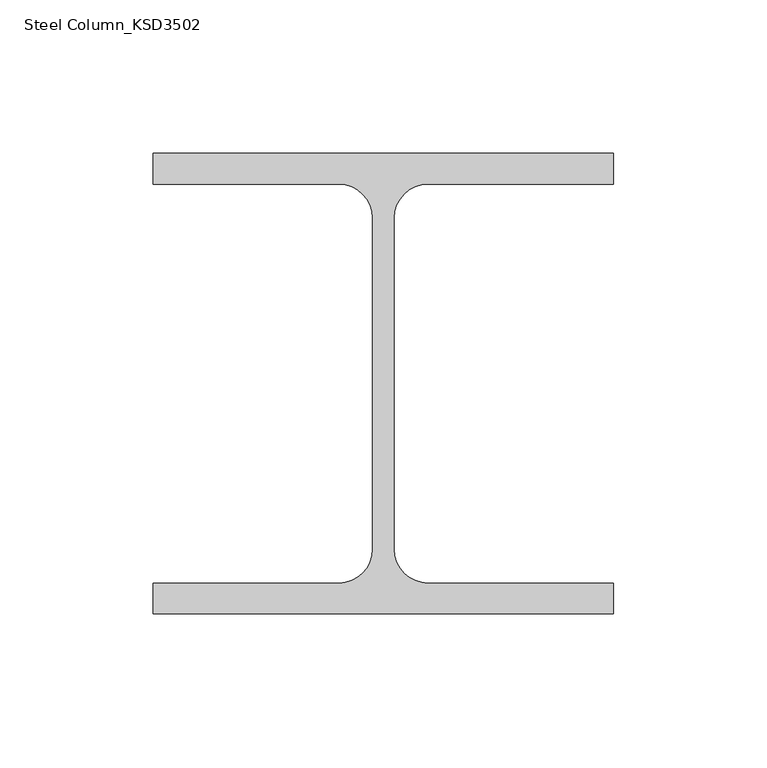
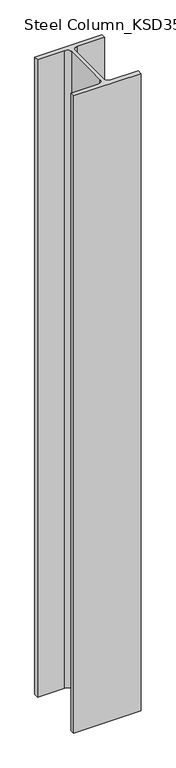
"""IFC4 building model written with IfcOpenShell, lengths in millimetres: column geometry, Steel Column_KSD3502 : H_SC_ASC_H-150×150x7x10."""

from ifc_helpers import new_model, si_unit, point, frame, frame_2d, origin, place, context, project, spatial, polyline, circle_curve, trimmed, segment, composite_curve, outline, extrude, source, transform, mapped, element, save


def steel_column_ksd3502_24869f1c(model_context):
    return source(origin(), model_context, "Body", "SweptSolid", [
        extrude(outline(composite_curve([segment(polyline([(75.0, 75.0), (75.0, 65.0), (14.5, 65.0)]), True, "CONTINUOUS"), segment(trimmed(circle_curve(frame_2d((14.5, 54.0)), 11.0), [point((14.5, 65.0))], [point((3.5, 54.0))], True, "CARTESIAN"), True, "CONTINUOUS"), segment(polyline([(3.5, 54.0), (3.5, -54.0)]), True, "CONTINUOUS"), segment(trimmed(circle_curve(frame_2d((14.5, -54.0)), 11.0), [point((3.5, -54.0))], [point((14.5, -65.0))], True, "CARTESIAN"), True, "CONTINUOUS"), segment(polyline([(14.5, -65.0), (75.0, -65.0), (75.0, -75.0), (-75.0, -75.0), (-75.0, -65.0), (-14.5, -65.0)]), True, "CONTINUOUS"), segment(trimmed(circle_curve(frame_2d((-14.5, -54.0)), 11.0), [point((-14.5, -65.0))], [point((-3.5, -54.0))], True, "CARTESIAN"), True, "CONTINUOUS"), segment(polyline([(-3.5, -54.0), (-3.5, 54.0)]), True, "CONTINUOUS"), segment(trimmed(circle_curve(frame_2d((-14.5, 54.0)), 11.0), [point((-3.5, 54.0))], [point((-14.5, 65.0))], True, "CARTESIAN"), True, "CONTINUOUS"), segment(polyline([(-14.5, 65.0), (-75.0, 65.0), (-75.0, 75.0), (75.0, 75.0)]), True, "CONTINUOUS")], self_intersect=False)), frame((0.0, 0.0, 17299.9720055), z_axis=(0.0, 0.0, 1.0), x_axis=(1.0, 0.0, 0.0)), (0.0, 0.0, 1.0), 1500.0),
    ])


if __name__ == "__main__":
    model = new_model("IFC4")
    model_context = context("Model", 3, world=origin())
    ifc_project = project(units=[si_unit("LENGTHUNIT", "METRE", prefix="MILLI")], contexts=[model_context])
    site = spatial("IfcSite", under=ifc_project)
    building = spatial("IfcBuilding", under=site)
    placement = place(None, origin())
    steel_column_ksd3502_shape = steel_column_ksd3502_24869f1c(model_context)
    element("IfcColumn", 1, ObjectType="Steel Column_KSD3502 : H_SC_ASC_H-150×150x7x10", at=placement, inside=building, context=model_context, shape_type="MappedRepresentation", body=[
        mapped(steel_column_ksd3502_shape, transform((0.0, 0.0, 0.0), x_axis=(1.0, 0.0, 0.0), y_axis=(0.0, 1.0, 0.0), z_axis=(0.0, 0.0, 1.0))),
    ])
    save(model, "model.ifc")

# Revit data of these elements
# Type "Steel Column_KSD3502 : H_SC_ASC_H-150×150x7x10"
#   Width = 15.0 cm
#   Web Thickness = 0.7 cm
#   Web Fillet = 1.1 cm
#   Warping Constant = 27562.5 cm⁶
#   Torsional Moment of Inertia = 11.6007 cm⁴
#   Section Area = 40.14 cm²
#   Plastic Modulus weak axis = 115.0 cm³
#   Plastic Modulus strong axis = 246.0 cm³
#   Perimeter = 1.27 m²/m
#   Nominal Weight = 31.50 kgf/m
#   Moment of Inertia weak axis = 563.00 cm⁴
#   Moment of Inertia strong axis = 1640.00 cm⁴
#   Height = 15.0 cm
#   Flange Thickness = 1.0 cm
#   Elastic Modulus weak axis = 75.1 cm³
#   Elastic Modulus strong axis = 219.0 cm³
#   Centroid Vertical = 7.5 cm
#   Centroid Horizontal = 7.5 cm
#   Bolt Spacing = 13.97 cm
#   Structural Material [instance default] = Steel, 45-345
#   Section Name Key = ""
#   Assembly Code = ""
# Element 1 (IfcColumn, "Steel Column_KSD3502 : H_SC_ASC_H-150×150x7x10")
#   Structural Material = none
# Materials
#   "Steel, 45-345": class "Metal", colour RGB 189 187 185, transparency 0, Description = "Steel 345 MPa", Cost = 0
